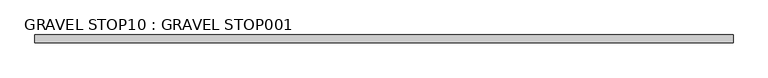
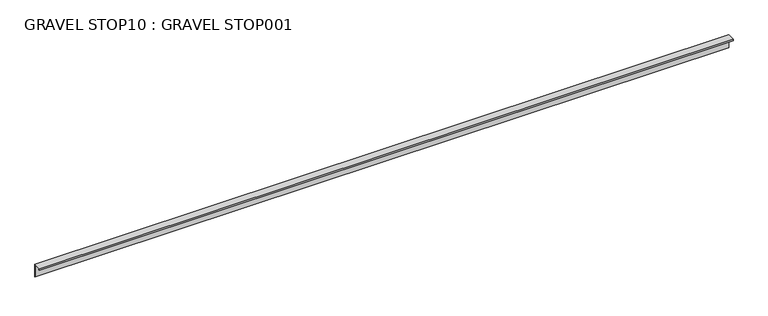
"""IFC4 building model written with IfcOpenShell, lengths in millimetres: proxy geometry, GRAVEL STOP10 : GRAVEL STOP001."""

import ifcopenshell
import ifcopenshell.guid

model = None  # the IFC model being written
_history = None  # IfcOwnerHistory: only IFC2X3 demands one
_inside = {}  # id of a spatial element -> (the spatial element, [elements in it])
_under = {}  # id of a project, library or spatial element -> (it, [spatial elements below it])
_declared = {}  # id of a project -> (the project, [libraries it declares])
_typed = {}  # id of a type object -> (the type object, [elements of that type])
_made_of = {}  # id of a material, layer set ... -> (it, [elements and type objects made of it])


def new_model(schema):
    """Start an empty IFC model of exactly this schema.

    Asked for "IFC4X3", IfcOpenShell would pick the latest addendum, in which some entities
    have other attributes; the version numbers below select the first issue.
    IFC2X3 requires an IfcOwnerHistory on every rooted entity: one is made here for all.
    """
    global model, _history
    if schema == "IFC4X3":
        model = ifcopenshell.file(schema_version=(4, 3, 0, 0))
    else:
        model = ifcopenshell.file(schema=schema)
    _inside.clear()
    _under.clear()
    _declared.clear()
    _typed.clear()
    _made_of.clear()
    _history = None
    if model.schema == "IFC2X3":
        org = make("IfcOrganization", Name="unknown")
        user = make(
            "IfcPersonAndOrganization",
            ThePerson=make("IfcPerson", FamilyName="unknown"),
            TheOrganization=org,
        )
        app = make(
            "IfcApplication",
            ApplicationDeveloper=org,
            Version="unknown",
            ApplicationFullName="unknown",
            ApplicationIdentifier="unknown",
        )
        _history = make(
            "IfcOwnerHistory",
            OwningUser=user,
            OwningApplication=app,
            ChangeAction="ADDED",
            CreationDate=0,
        )
    return model


def make(cls, **values):
    """One entity of the class cls with the attributes given. An attribute that is None is left unset."""
    return model.create_entity(
        cls, **{name: value for name, value in values.items() if value is not None}
    )


def rooted(cls, **values):
    """An entity with a GlobalId (a new one), such as an element, a storey or a relation."""
    return make(cls, GlobalId=ifcopenshell.guid.new(), OwnerHistory=_history, **values)


def si_unit(unit_type, name, prefix=None):
    """IfcSIUnit, for example si_unit("LENGTHUNIT", "METRE", prefix="MILLI")."""
    return make("IfcSIUnit", UnitType=unit_type, Prefix=prefix, Name=name)


def assignment(units):
    """IfcUnitAssignment: the units of a project."""
    return None if units is None else make("IfcUnitAssignment", Units=units)


def point(xyz):
    """IfcCartesianPoint."""
    return None if xyz is None else make("IfcCartesianPoint", Coordinates=xyz)


def direction(xyz):
    """IfcDirection."""
    return None if xyz is None else make("IfcDirection", DirectionRatios=xyz)


def frame(location, z_axis=None, x_axis=None):
    """IfcAxis2Placement3D, a coordinate frame: its origin and axes. An axis left out is left unset."""
    return make(
        "IfcAxis2Placement3D",
        Location=point(location),
        Axis=direction(z_axis),
        RefDirection=direction(x_axis),
    )


def origin():
    """The frame at (0, 0, 0) with its axes left unset."""
    return frame((0.0, 0.0, 0.0))


def place(relative_to, where):
    """IfcLocalPlacement: puts the frame where relative to a parent placement (None: the world)."""
    return make(
        "IfcLocalPlacement", PlacementRelTo=relative_to, RelativePlacement=where
    )


def context(
    kind, dimensions, precision=None, world=None, true_north=None, identifier=None
):
    """IfcGeometricRepresentationContext, for example the 3D "Model" context."""
    return make(
        "IfcGeometricRepresentationContext",
        ContextIdentifier=identifier,
        ContextType=kind,
        CoordinateSpaceDimension=dimensions,
        Precision=precision,
        WorldCoordinateSystem=world,
        TrueNorth=true_north,
    )


def project(units=None, contexts=None):
    """IfcProject with its units and contexts."""
    return rooted(
        "IfcProject",
        Name="project",
        RepresentationContexts=contexts,
        UnitsInContext=assignment(units),
    )


def spatial(cls, under=None, at=None, **own):
    """A site, building, storey or space (cls), placed at a placement, below another one or the project."""
    s = rooted(cls, ObjectPlacement=at, **own)
    if under is not None:
        _under.setdefault(under.id(), (under, []))[1].append(s)
    return s


def polyline(points):
    """IfcPolyline through the points."""
    return make("IfcPolyline", Points=[point(p) for p in points])


def outline(outer, holes=None, kind="AREA"):
    """IfcArbitraryClosedProfileDef: a profile drawn as a closed curve; with holes, ...WithVoids."""
    if holes is None:
        return make("IfcArbitraryClosedProfileDef", ProfileType=kind, OuterCurve=outer)
    return make(
        "IfcArbitraryProfileDefWithVoids",
        ProfileType=kind,
        OuterCurve=outer,
        InnerCurves=holes,
    )


def extrude(swept, where, along, depth):
    """IfcExtrudedAreaSolid: the profile swept, set in the frame where, extruded along a direction by depth."""
    return make(
        "IfcExtrudedAreaSolid",
        SweptArea=swept,
        Position=where,
        ExtrudedDirection=direction(along),
        Depth=depth,
    )


def shape(context_of_items, identifier, shape_type, items):
    """IfcShapeRepresentation: the items that make up one representation, for example the "Body"."""
    return make(
        "IfcShapeRepresentation",
        ContextOfItems=context_of_items,
        RepresentationIdentifier=identifier,
        RepresentationType=shape_type,
        Items=items,
    )


def source(mapping_origin, context_of_items, identifier, shape_type, items):
    """IfcRepresentationMap: a shape defined once, which mapped items show again and again."""
    return make(
        "IfcRepresentationMap",
        MappingOrigin=mapping_origin,
        MappedRepresentation=shape(context_of_items, identifier, shape_type, items),
    )


def transform(
    local_origin,
    x_axis=None,
    y_axis=None,
    z_axis=None,
    scale=None,
    scale2=None,
    scale3=None,
    uniform=True,
):
    """IfcCartesianTransformationOperator3D, or its non-uniform kind. x_axis, y_axis, z_axis: its Axis1, 2, 3."""
    if uniform:
        return make(
            "IfcCartesianTransformationOperator3D",
            Axis1=direction(x_axis),
            Axis2=direction(y_axis),
            LocalOrigin=point(local_origin),
            Scale=scale,
            Axis3=direction(z_axis),
        )
    return make(
        "IfcCartesianTransformationOperator3DnonUniform",
        Axis1=direction(x_axis),
        Axis2=direction(y_axis),
        LocalOrigin=point(local_origin),
        Scale=scale,
        Axis3=direction(z_axis),
        Scale2=scale2,
        Scale3=scale3,
    )


def mapped(mapping_source, mapping_target):
    """IfcMappedItem: shows the shape of a source again, moved by a transform."""
    return make(
        "IfcMappedItem", MappingSource=mapping_source, MappingTarget=mapping_target
    )


def made_of(thing, what):
    """Note that an element or type object is made of a material, layer set ...; save() writes the relation."""
    if what is not None:
        _made_of.setdefault(what.id(), (what, []))[1].append(thing)
    return thing


def element(
    cls,
    number,
    at=None,
    inside=None,
    cuts=None,
    type_object=None,
    material=None,
    context=None,
    identifier="Body",
    shape_type=None,
    held_by="IfcProductDefinitionShape",
    body=None,
    shapes=None,
    **own,
):
    """One element of the class cls, such as IfcWall. Its Tag is "e" and its number.

    at: its placement. inside: the storey or other place that contains it. cuts: it is an
    opening in that element (IfcRelVoidsElement). A single representation is given by context,
    identifier, shape_type and body (its items); several are given by shapes. held_by: the class
    of the entity that holds the representations. save() writes the other relations.
    """
    e = rooted(cls, Tag="e%d" % number, ObjectPlacement=at, **own)
    if body is not None:
        shapes = [shape(context, identifier, shape_type, body)]
    if shapes is not None:
        e.Representation = make(held_by, Representations=shapes)
    if inside is not None:
        _inside.setdefault(inside.id(), (inside, []))[1].append(e)
    if cuts is not None:
        rooted(
            "IfcRelVoidsElement", RelatingBuildingElement=cuts, RelatedOpeningElement=e
        )
    if type_object is not None:
        _typed.setdefault(type_object.id(), (type_object, []))[1].append(e)
    return made_of(e, material)


def aggregate(whole, parts):
    """IfcRelAggregates: a whole, such as a stair, and the parts it consists of."""
    return rooted("IfcRelAggregates", RelatingObject=whole, RelatedObjects=parts)


def save(model, path):
    """Write the relations noted so far, then the file.

    IfcRelAggregates (storeys below a building ...), IfcRelContainedInSpatialStructure (elements
    in a storey), IfcRelDefinesByType, IfcRelAssociatesMaterial and IfcRelDeclares: one each for
    every whole, place, type object, material and project.
    """
    for whole, parts in _under.values():
        aggregate(whole, parts)
    for where, things in _inside.values():
        rooted(
            "IfcRelContainedInSpatialStructure",
            RelatedElements=things,
            RelatingStructure=where,
        )
    for kind, things in _typed.values():
        rooted("IfcRelDefinesByType", RelatedObjects=things, RelatingType=kind)
    for what, things in _made_of.values():
        rooted("IfcRelAssociatesMaterial", RelatedObjects=things, RelatingMaterial=what)
    for by, libraries in _declared.values():
        rooted("IfcRelDeclares", RelatingContext=by, RelatedDefinitions=libraries)
    model.write(path)


def gravel_stop10_gravel_stop001_c600786e(model_context):
    return source(origin(), model_context, "Body", "SweptSolid", [
        extrude(outline(polyline([(-5562.4629675, 40210.7296087), (-5582.1479675, 40210.7296087), (-5582.1479675, 40208.5198087), (-5580.4155111, 40208.5198087), (-5580.4155111, 40207.2498087), (-5583.4179675, 40207.2498087), (-5583.4179675, 40211.9996087), (-5561.1929675, 40211.9996087), (-5561.1929675, 40173.8996087), (-5562.4629675, 40173.8996087), (-5562.4629675, 40210.7296087)])), frame((12382.7678845, 0.0, 0.0), z_axis=(1.0, 0.0, 0.0), x_axis=(0.0, 1.0, 0.0)), (0.0, 0.0, 1.0), 2000.25),
    ])


if __name__ == "__main__":
    model = new_model("IFC4")
    model_context = context("Model", 3, world=origin())
    ifc_project = project(units=[si_unit("LENGTHUNIT", "METRE", prefix="MILLI")], contexts=[model_context])
    site = spatial("IfcSite", under=ifc_project)
    building = spatial("IfcBuilding", under=site)
    placement = place(None, origin())
    gravel_stop10_gravel_stop001_shape = gravel_stop10_gravel_stop001_c600786e(model_context)
    element("IfcBuildingElementProxy", 1, Name="GRAVEL STOP10 : GRAVEL STOP001", ObjectType="GRAVEL STOP10 : GRAVEL STOP001", at=placement, inside=building, context=model_context, shape_type="MappedRepresentation", body=[
        mapped(gravel_stop10_gravel_stop001_shape, transform((0.0, 0.0, 0.0), x_axis=(1.0, 0.0, 0.0), y_axis=(0.0, 1.0, 0.0), z_axis=(0.0, 0.0, 1.0))),
    ])
    save(model, "model.ifc")

# Revit data of these elements
# Type "GRAVEL STOP10 : GRAVEL STOP001"
#   NameOverride = "GRAVEL STOP001"
# Element 1 (IfcBuildingElementProxy, "GRAVEL STOP10 : GRAVEL STOP001")
#   Materials on its faces: "COPPER STUCCO J BEAD"
# Materials
#   "COPPER STUCCO J BEAD": class "Unassigned", colour RGB 251 232 155, transparency 0, Cost = 0
